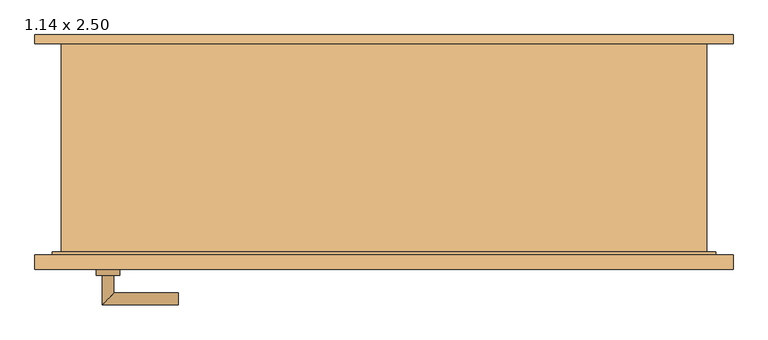
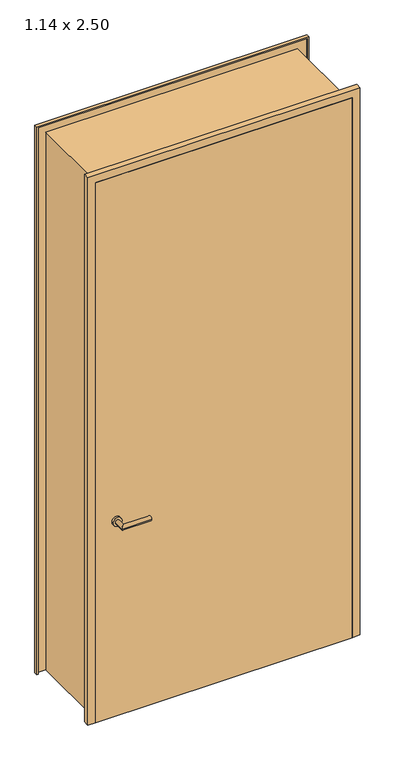
"""IFC4 building model written with IfcOpenShell, lengths in millimetres: door geometry, Drehflügel 1-flg - Stahlzarge : 1.14 x 2.50."""

from ifc_helpers import new_model, si_unit, point, frame, frame_2d, origin, place, context, project, spatial, polyline, circle_curve, ellipse_curve, trimmed, segment, composite_curve, outline, extrude, faceted_brep, source, transform, mapped, element, save
from ifc_brep_helpers import plane_surface, cylinder_surface, advanced_brep


def door_1_14_x_2_50_3de6b391(model_context):
    return source(origin(), model_context, "Body", "SolidModel", [
        advanced_brep(
        [(-480.0, -169.4346141, 915.0), (-460.0, -169.4346141, 915.0), (-460.0, -119.4346141, 915.0), (-480.0, -99.4346141, 915.0), (-350.0, -99.4346141, 915.0), (-350.0, -119.4346141, 915.0)],
        [
            (0, 1, circle_curve(frame((-470.0, -169.4346141, 915.0), z_axis=(0.0, -1.0, 0.0), x_axis=(1.0, 0.0, 0.0)), 10.0)),
            (1, 0, circle_curve(frame((-470.0, -169.4346141, 915.0), z_axis=(0.0, -1.0, 0.0), x_axis=(1.0, 0.0, 0.0)), 10.0)),
            (1, 2),
            (2, 3, ellipse_curve(frame((-470.0, -109.4346141, 915.0), z_axis=(-0.7071067811865385, -0.7071067811865565, 0.0), x_axis=(0.7071067811865563, -0.7071067811865386, 0.0)), 14.1421356, 10.0)),
            (3, 0),
            (3, 2, ellipse_curve(frame((-470.0, -109.4346141, 915.0), z_axis=(-0.7071067811865385, -0.7071067811865565, 0.0), x_axis=(0.7071067811865563, -0.7071067811865386, 0.0)), 14.1421356, 10.0)),
            (4, 5, circle_curve(frame((-350.0, -109.4346141, 915.0), z_axis=(1.0, 0.0, 0.0), x_axis=(0.0, -1.0, 0.0)), 10.0)),
            (5, 4, circle_curve(frame((-350.0, -109.4346141, 915.0), z_axis=(1.0, 0.0, 0.0), x_axis=(0.0, -1.0, 0.0)), 10.0)),
            (2, 5),
            (4, 3),
        ],
        [
            plane_surface(frame((-470.0, -169.4346141, -372.7526403), z_axis=(0.0, -1.0, 0.0), x_axis=(0.0, 0.0, 1.0))),
            cylinder_surface(frame((-470.0, -169.4346141, 915.0), z_axis=(0.0, -1.0, 0.0), x_axis=(1.0, 0.0, 0.0)), 10.0),
            plane_surface(frame((-350.0, -109.4346141, -372.7526403), z_axis=(1.0, 0.0, 0.0), x_axis=(0.0, 0.0, 1.0))),
            cylinder_surface(frame((-470.0, -109.4346141, 915.0), z_axis=(-1.0, 0.0, 0.0), x_axis=(0.0, -1.0, 0.0)), 10.0),
        ],
        [
            (0, [[1, 2]]),
            (1, [[3, 4, 5, -2]]),
            (1, [[-5, 6, -3, -1]]),
            (2, [[7, 8]]),
            (3, [[9, -7, 10, -4]]),
            (3, [[-10, -8, -9, -6]]),
        ],
    ),
        advanced_brep(
        [(-460.0, -229.4346141, 915.0), (-480.0, -229.4346141, 915.0), (-480.0, -279.4346141, 915.0), (-460.0, -259.4346141, 915.0), (-350.0, -259.4346141, 915.0), (-350.0, -279.4346141, 915.0)],
        [
            (0, 1, circle_curve(frame((-470.0, -229.4346141, 915.0), z_axis=(0.0, 1.0, 0.0), x_axis=(-1.0, 0.0, 0.0)), 10.0)),
            (1, 0, circle_curve(frame((-470.0, -229.4346141, 915.0), z_axis=(0.0, 1.0, 0.0), x_axis=(-1.0, 0.0, 0.0)), 10.0)),
            (1, 2),
            (2, 3, ellipse_curve(frame((-470.0, -269.4346141, 915.0), z_axis=(-0.7071067811865475, 0.7071067811865475, 0.0), x_axis=(0.7071067811865474, 0.7071067811865476, 0.0)), 14.1421356, 10.0)),
            (3, 0),
            (3, 2, ellipse_curve(frame((-470.0, -269.4346141, 915.0), z_axis=(-0.7071067811865475, 0.7071067811865475, 0.0), x_axis=(0.7071067811865474, 0.7071067811865476, 0.0)), 14.1421356, 10.0)),
            (4, 5, circle_curve(frame((-350.0, -269.4346141, 915.0), z_axis=(1.0, 0.0, 0.0), x_axis=(0.0, -1.0, 0.0)), 10.0)),
            (5, 4, circle_curve(frame((-350.0, -269.4346141, 915.0), z_axis=(1.0, 0.0, 0.0), x_axis=(0.0, -1.0, 0.0)), 10.0)),
            (2, 5),
            (4, 3),
        ],
        [
            plane_surface(frame((-470.0, -229.4346141, -372.7526403), z_axis=(0.0, 1.0, 0.0), x_axis=(0.0, 0.0, 1.0))),
            cylinder_surface(frame((-470.0, -229.4346141, 915.0), z_axis=(0.0, 1.0, 0.0), x_axis=(-1.0, 0.0, 0.0)), 10.0),
            plane_surface(frame((-350.0, -269.4346141, -372.7526403), z_axis=(1.0, 0.0, 0.0), x_axis=(0.0, 0.0, 1.0))),
            cylinder_surface(frame((-470.0, -269.4346141, 915.0), z_axis=(-1.0, 0.0, 0.0), x_axis=(0.0, -1.0, 0.0)), 10.0),
        ],
        [
            (0, [[1, 2]]),
            (1, [[3, 4, 5, -2]]),
            (1, [[-5, 6, -3, -1]]),
            (2, [[7, 8]]),
            (3, [[9, -7, 10, -4]]),
            (3, [[-10, -8, -9, -6]]),
        ],
    ),
        extrude(outline(composite_curve([segment(trimmed(circle_curve(frame_2d((915.0, -470.0)), 20.0), [point((915.0, -490.0))], [point((915.0, -450.0))], False, "CARTESIAN"), True, "CONTINUOUS"), segment(trimmed(circle_curve(frame_2d((915.0, -470.0)), 20.0), [point((915.0, -450.0))], [point((915.0, -490.0))], False, "CARTESIAN"), True, "CONTINUOUS")], self_intersect=False)), frame((0.0, -169.4346141, 0.0), z_axis=(0.0, 1.0, 0.0), x_axis=(0.0, 0.0, 1.0)), (0.0, 0.0, 1.0), 10.0),
        extrude(outline(composite_curve([segment(trimmed(circle_curve(frame_2d((915.0, -470.0)), 20.0), [point((915.0, -490.0))], [point((915.0, -450.0))], False, "CARTESIAN"), True, "CONTINUOUS"), segment(trimmed(circle_curve(frame_2d((915.0, -470.0)), 20.0), [point((915.0, -450.0))], [point((915.0, -490.0))], False, "CARTESIAN"), True, "CONTINUOUS")], self_intersect=False)), frame((0.0, -229.4346141, 0.0), z_axis=(0.0, 1.0, 0.0), x_axis=(0.0, 0.0, 1.0)), (0.0, 0.0, 1.0), 10.0),
        extrude(outline(polyline([(560.0, -194.4346141), (560.0, -219.4346141), (-560.0, -219.4346141), (-560.0, -194.4346141), (560.0, -194.4346141)])), frame((0.0, 0.0, 15.0), z_axis=(0.0, 0.0, 1.0), x_axis=(1.0, 0.0, 0.0)), (0.0, 0.0, 1.0), 2490.0),
        faceted_brep([(594.4603207, 180.5653859, 15.0), (594.4603207, 165.5653859, 15.0), (589.4603207, 165.5653859, 15.0), (589.4603207, 175.5653859, 15.0), (550.0, 175.5653859, 15.0), (550.0, -189.4346141, 15.0), (565.0, -189.4346141, 15.0), (565.0, -214.4346141, 15.0), (589.4603207, -214.4346141, 15.0), (589.4603207, -194.4346141, 15.0), (594.4603207, -194.4346141, 15.0), (594.4603207, -219.4346141, 15.0), (560.0, -219.4346141, 15.0), (560.0, -194.4346141, 15.0), (545.0, -194.4346141, 15.0), (545.0, 180.5653859, 15.0), (545.0, 180.5653859, 2490.0), (-545.0, 180.5653859, 2490.0), (-545.0, 180.5653859, 15.0), (-594.4603207, 180.5653859, 15.0), (-594.4603207, 180.5653859, 2539.4603207), (594.4603207, 180.5653859, 2539.4603207), (545.0, -194.4346141, 2490.0), (560.0, -194.4346141, 2505.0), (-560.0, -194.4346141, 2505.0), (-560.0, -194.4346141, 15.0), (-545.0, -194.4346141, 15.0), (-545.0, -194.4346141, 2490.0), (560.0, -219.4346141, 2505.0), (594.4603207, -219.4346141, 2539.4603207), (-594.4603207, -219.4346141, 2539.4603207), (-594.4603207, -219.4346141, 15.0), (-560.0, -219.4346141, 15.0), (-560.0, -219.4346141, 2505.0), (594.4603207, -194.4346141, 2539.4603207), (589.4603207, -194.4346141, 2534.4603207), (-589.4603207, -194.4346141, 2534.4603207), (-589.4603207, -194.4346141, 15.0), (-594.4603207, -194.4346141, 15.0), (-594.4603207, -194.4346141, 2539.4603207), (589.4603207, -214.4346141, 2534.4603207), (565.0, -214.4346141, 2510.0), (-565.0, -214.4346141, 2510.0), (-565.0, -214.4346141, 15.0), (-589.4603207, -214.4346141, 15.0), (-589.4603207, -214.4346141, 2534.4603207), (565.0, -189.4346141, 2510.0), (550.0, -189.4346141, 2495.0), (-550.0, -189.4346141, 2495.0), (-550.0, -189.4346141, 15.0), (-565.0, -189.4346141, 15.0), (-565.0, -189.4346141, 2510.0), (550.0, 175.5653859, 2495.0), (589.4603207, 175.5653859, 2534.4603207), (-589.4603207, 175.5653859, 2534.4603207), (-589.4603207, 175.5653859, 15.0), (-550.0, 175.5653859, 15.0), (-550.0, 175.5653859, 2495.0), (589.4603207, 165.5653859, 2534.4603207), (594.4603207, 165.5653859, 2539.4603207), (-594.4603207, 165.5653859, 2539.4603207), (-594.4603207, 165.5653859, 15.0), (-589.4603207, 165.5653859, 15.0), (-589.4603207, 165.5653859, 2534.4603207)], [[[0, 1, 2, 3, 4, 5, 6, 7, 8, 9, 10, 11, 12, 13, 14, 15]], [[15, 16, 17, 18, 19, 20, 21, 0]], [[14, 22, 16, 15]], [[13, 23, 24, 25, 26, 27, 22, 14]], [[12, 28, 23, 13]], [[11, 29, 30, 31, 32, 33, 28, 12]], [[10, 34, 29, 11]], [[9, 35, 36, 37, 38, 39, 34, 10]], [[8, 40, 35, 9]], [[7, 41, 42, 43, 44, 45, 40, 8]], [[6, 46, 41, 7]], [[5, 47, 48, 49, 50, 51, 46, 6]], [[4, 52, 47, 5]], [[3, 53, 54, 55, 56, 57, 52, 4]], [[2, 58, 53, 3]], [[1, 59, 60, 61, 62, 63, 58, 2]], [[0, 21, 59, 1]], [[20, 19, 61, 60]], [[19, 18, 26, 25, 32, 31, 38, 37, 44, 43, 50, 49, 56, 55, 62, 61]], [[27, 26, 18, 17]], [[33, 32, 25, 24]], [[39, 38, 31, 30]], [[45, 44, 37, 36]], [[51, 50, 43, 42]], [[57, 56, 49, 48]], [[63, 62, 55, 54]], [[22, 27, 17, 16]], [[28, 33, 24, 23]], [[34, 39, 30, 29]], [[40, 45, 36, 35]], [[46, 51, 42, 41]], [[52, 57, 48, 47]], [[58, 63, 54, 53]], [[21, 20, 60, 59]]]),
    ])


if __name__ == "__main__":
    model = new_model("IFC4")
    model_context = context("Model", 3, world=origin())
    ifc_project = project(units=[si_unit("LENGTHUNIT", "METRE", prefix="MILLI")], contexts=[model_context])
    site = spatial("IfcSite", under=ifc_project)
    building = spatial("IfcBuilding", under=site)
    placement = place(None, origin())
    door_1_14_x_2_50_shape = door_1_14_x_2_50_3de6b391(model_context)
    element("IfcDoor", 1, ObjectType="Drehflügel 1-flg - Stahlzarge : 1.14 x 2.50", at=placement, inside=building, context=model_context, shape_type="MappedRepresentation", body=[
        mapped(door_1_14_x_2_50_shape, transform((0.0, 0.0, 0.0), x_axis=(1.0, 0.0, 0.0), y_axis=(0.0, 1.0, 0.0), z_axis=(0.0, 0.0, 1.0))),
    ])
    save(model, "model.ifc")

# Revit data of these elements
# Type "Drehflügel 1-flg - Stahlzarge : 1.14 x 2.50"
#   Type Mark = "28"
#   Operation = "SingleSwingRight"
#   Keynote = "16.03"
#   Analytic Construction = "Metall"
#   Thermal Resistance (R) = 0.270117 (m²·K)/W
#   Heat Transfer Coefficient (U) = 3.7021 W/(m²·K)
#   Rough Width = 1.140 m
#   Rough Height [instance default] = 2.600 m
#   Höhe Türgriff [instance default] = 0.900 m
#   Height = 2.500 m
#   Fußbodenaufbau [instance default] = 0.100 m
#   Width = 1.140 m
#   Sichtbarkeit Sturzlinien [instance default] = yes
#   Türgriff auswählen [instance default] = element 221079
#   Türgriff [instance default] = none
#   Türflügel [instance default] = none
#   Rahmen/Pfosten [instance default] = Metall - Lackiert - Grau
#   Visual Light Transmittance = 0
#   Solar Heat Gain Coefficient = 0
#   Function = (empty or 0)
#   Wall Closure = (empty or 0)
# Element 1 (IfcDoor, "Drehflügel 1-flg - Stahlzarge : 1.14 x 2.50")
#   Rough Height = 2.515 m
#   Fußbodenaufbau = 0.015 m
#   Materials on its faces: "Metall - Lackiert - Grau", "Metall - Chrom", "Holz - Birke"
# Materials
#   "Metall - Lackiert - Grau": class "Farbe 1", colour RGB 98 98 98, transparency 0, Cost = 0
#   "Metall - Chrom": class "Metall", colour RGB 247 247 247, transparency 0, Cost = 0
#   "Holz - Birke": class "Holz", colour RGB 213 164 103, transparency 0, Cost = 0
